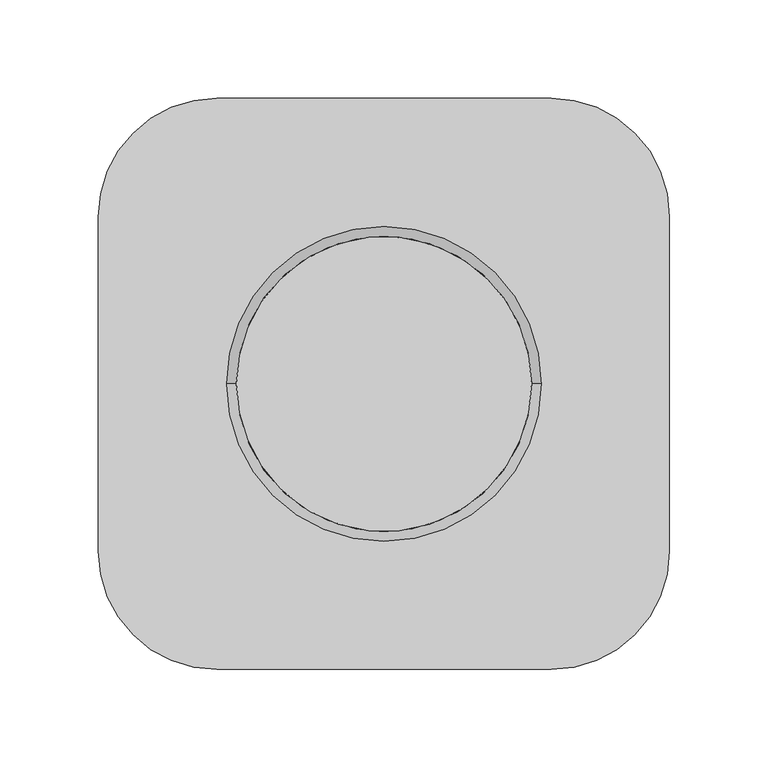
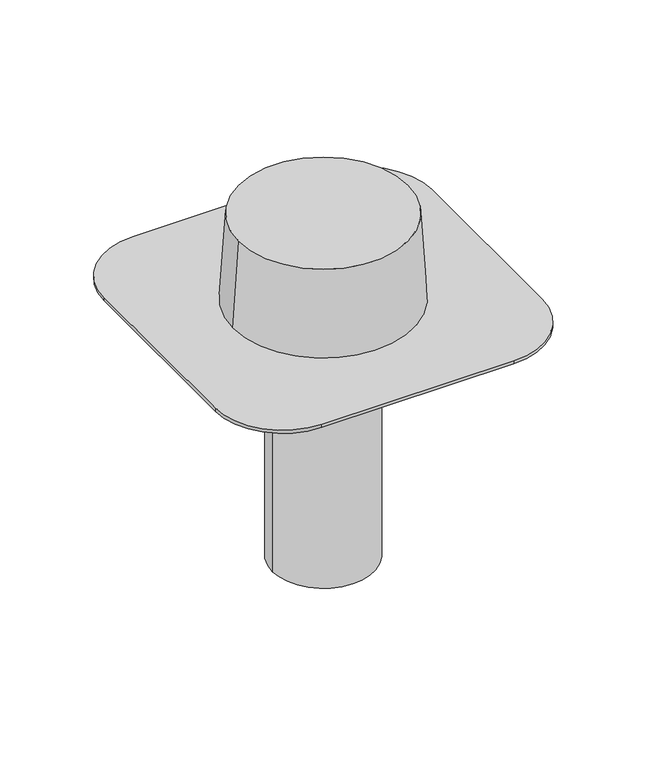
"""IFC4 building model written with IfcOpenShell, lengths in millimetres: proxy geometry, TN_Воронка ТехноНИКОЛЬ ремонтная : Воронка ТехноНИКОЛЬ ремонтная, 90Х240."""

from ifc_helpers import new_model, si_unit, frame, origin, place, context, project, spatial, polyline, circle_curve, source, transform, mapped, element, save
from ifc_brep_helpers import plane_surface, cylinder_surface, revolved_surface, advanced_brep


def specialty_equipment_9be2945b(model_context):
    return source(origin(), model_context, "Body", "AdvancedBrep", [
        advanced_brep(
        [(0.0, 0.0, -240.0), (-45.0, 0.0, -240.0), (45.0, 0.0, -240.0), (-45.0, 0.0, -3.0), (45.0, 0.0, -3.0), (85.0, 145.0, -3.0), (145.0, 85.0, -3.0), (145.0, -85.0, -3.0), (85.0, -145.0, -3.0), (-85.0, -145.0, -3.0), (-145.0, -85.0, -3.0), (-145.0, 85.0, -3.0), (-85.0, 145.0, -3.0), (85.0, 145.0, 0.0), (-85.0, 145.0, 0.0), (-145.0, 85.0, 0.0), (-145.0, -85.0, 0.0), (-85.0, -145.0, 0.0), (85.0, -145.0, 0.0), (145.0, -85.0, 0.0), (145.0, 85.0, 0.0)],
        [
            (0, 1),
            (1, 2, circle_curve(frame((0.0, 0.0, -240.0), z_axis=(0.0, 0.0, -1.0), x_axis=(-1.0, 0.0, 0.0)), 45.0)),
            (2, 0),
            (2, 1, circle_curve(frame((0.0, 0.0, -240.0), z_axis=(0.0, 0.0, -1.0), x_axis=(-1.0, 0.0, 0.0)), 45.0)),
            (1, 3),
            (3, 4, circle_curve(frame((0.0, 0.0, -3.0), z_axis=(0.0, 0.0, -1.0), x_axis=(-1.0, 0.0, 0.0)), 45.0)),
            (4, 2),
            (4, 3, circle_curve(frame((0.0, 0.0, -3.0), z_axis=(0.0, 0.0, -1.0), x_axis=(-1.0, 0.0, 0.0)), 45.0)),
            (5, 6, circle_curve(frame((85.0, 85.0, -3.0), z_axis=(0.0, 0.0, -1.0), x_axis=(1.0, 0.0, 0.0)), 60.0)),
            (6, 7),
            (7, 8, circle_curve(frame((85.0, -85.0, -3.0), z_axis=(0.0, 0.0, -1.0), x_axis=(1.0, 0.0, 0.0)), 60.0)),
            (8, 9),
            (9, 10, circle_curve(frame((-85.0, -85.0, -3.0), z_axis=(0.0, 0.0, -1.0), x_axis=(1.0, 0.0, 0.0)), 60.0)),
            (10, 11),
            (11, 12, circle_curve(frame((-85.0, 85.0, -3.0), z_axis=(0.0, 0.0, -1.0), x_axis=(1.0, 0.0, 0.0)), 60.0)),
            (12, 5),
            (13, 14),
            (14, 15, circle_curve(frame((-85.0, 85.0, 0.0), z_axis=(0.0, 0.0, 1.0), x_axis=(1.0, 0.0, 0.0)), 60.0)),
            (15, 16),
            (16, 17, circle_curve(frame((-85.0, -85.0, 0.0), z_axis=(0.0, 0.0, 1.0), x_axis=(1.0, 0.0, 0.0)), 60.0)),
            (17, 18),
            (18, 19, circle_curve(frame((85.0, -85.0, 0.0), z_axis=(0.0, 0.0, 1.0), x_axis=(1.0, 0.0, 0.0)), 60.0)),
            (19, 20),
            (20, 13, circle_curve(frame((85.0, 85.0, 0.0), z_axis=(0.0, 0.0, 1.0), x_axis=(1.0, 0.0, 0.0)), 60.0)),
            (12, 14),
            (13, 5),
            (10, 16),
            (15, 11),
            (8, 18),
            (17, 9),
            (6, 20),
            (19, 7),
        ],
        [
            plane_surface(frame((0.0, 0.0, -240.0), z_axis=(0.0, 0.0, -1.0), x_axis=(-1.0, 0.0, 0.0))),
            cylinder_surface(frame((0.0, 0.0, 0.0), z_axis=(0.0, 0.0, -1.0), x_axis=(-1.0, 0.0, 0.0)), 45.0),
            plane_surface(frame((-350.0, 145.0, -3.0), z_axis=(0.0, 0.0, -1.0), x_axis=(1.0, 0.0, 0.0))),
            plane_surface(frame((-350.0, 145.0, 0.0), z_axis=(0.0, 0.0, 1.0), x_axis=(-1.0, 0.0, 0.0))),
            plane_surface(frame((85.0, 145.0, 0.0), z_axis=(0.0, 1.0, 0.0), x_axis=(0.0, 0.0, -1.0))),
            plane_surface(frame((-145.0, 85.0, 0.0), z_axis=(-1.0, 0.0, 0.0), x_axis=(0.0, 0.0, -1.0))),
            plane_surface(frame((-85.0, -145.0, 0.0), z_axis=(0.0, -1.0, 0.0), x_axis=(0.0, 0.0, -1.0))),
            plane_surface(frame((145.0, -85.0, 0.0), z_axis=(1.0, 0.0, 0.0), x_axis=(0.0, 0.0, -1.0))),
            cylinder_surface(frame((-85.0, 85.0, -3.0), z_axis=(0.0, 0.0, 1.0), x_axis=(1.0, 0.0, 0.0)), 60.0),
            cylinder_surface(frame((-85.0, -85.0, -3.0), z_axis=(0.0, 0.0, 1.0), x_axis=(1.0, 0.0, 0.0)), 60.0),
            cylinder_surface(frame((85.0, -85.0, -3.0), z_axis=(0.0, 0.0, 1.0), x_axis=(1.0, 0.0, 0.0)), 60.0),
            cylinder_surface(frame((85.0, 85.0, -3.0), z_axis=(0.0, 0.0, 1.0), x_axis=(1.0, 0.0, 0.0)), 60.0),
        ],
        [
            (0, [[1, 2, 3]]),
            (0, [[-1, -3, 4]]),
            (1, [[-2, 5, 6, 7]]),
            (1, [[-4, -7, 8, -5]]),
            (2, [[9, 10, 11, 12, 13, 14, 15, 16], [-6, -8]]),
            (3, [[17, 18, 19, 20, 21, 22, 23, 24]]),
            (4, [[-16, 25, -17, 26]]),
            (5, [[-14, 27, -19, 28]]),
            (6, [[-12, 29, -21, 30]]),
            (7, [[-10, 31, -23, 32]]),
            (8, [[-15, -28, -18, -25]]),
            (9, [[-13, -30, -20, -27]]),
            (10, [[-11, -32, -22, -29]]),
            (11, [[-9, -26, -24, -31]]),
        ],
    ),
        advanced_brep(
        [(-75.0, 0.0, 80.0), (75.0, 0.0, 80.0), (-80.0, 0.0, 0.0), (80.0, 0.0, 0.0)],
        [
            (0, 1, circle_curve(frame((0.0, 0.0, 80.0), z_axis=(0.0, 0.0, 1.0), x_axis=(-1.0, 0.0, 0.0)), 75.0)),
            (1, 0, circle_curve(frame((0.0, 0.0, 80.0), z_axis=(0.0, 0.0, 1.0), x_axis=(1.0, 0.0, 0.0)), 75.0)),
            (2, 3, circle_curve(frame((0.0, 0.0, 0.0), z_axis=(0.0, 0.0, -1.0), x_axis=(1.0, 0.0, 0.0)), 80.0)),
            (3, 2, circle_curve(frame((0.0, 0.0, 0.0), z_axis=(0.0, 0.0, -1.0), x_axis=(-1.0, 0.0, 0.0)), 80.0)),
            (3, 1),
            (0, 2),
        ],
        [
            plane_surface(frame((0.0, 0.0, 80.0), z_axis=(0.0, 0.0, 1.0), x_axis=(0.0, -1.0, 0.0))),
            plane_surface(frame((0.0, 0.0, 0.0), z_axis=(0.0, 0.0, -1.0), x_axis=(0.0, -1.0, 0.0))),
            revolved_surface(polyline([(-75.0, 0.0, 80.0), (-80.0, 0.0, 0.0)]), (0.0, 0.0, 1280.0), (0.0, 0.0, -1.0)),
            revolved_surface(polyline([(75.0, 0.0, 80.0), (80.0, 0.0, 0.0)]), (0.0, 0.0, 1280.0), (0.0, 0.0, -1.0)),
        ],
        [
            (0, [[1, 2]]),
            (1, [[3, 4]]),
            (2, [[-4, 5, -1, 6]]),
            (3, [[-3, -6, -2, -5]]),
        ],
    ),
    ])


if __name__ == "__main__":
    model = new_model("IFC4")
    model_context = context("Model", 3, world=origin())
    ifc_project = project(units=[si_unit("LENGTHUNIT", "METRE", prefix="MILLI")], contexts=[model_context])
    site = spatial("IfcSite", under=ifc_project)
    building = spatial("IfcBuilding", under=site)
    placement = place(None, origin())
    specialty_equipment_shape = specialty_equipment_9be2945b(model_context)
    element("IfcBuildingElementProxy", 1, Name="TN_Воронка ТехноНИКОЛЬ ремонтная : Воронка ТехноНИКОЛЬ ремонтная, 90Х240", ObjectType="TN_Воронка ТехноНИКОЛЬ ремонтная : Воронка ТехноНИКОЛЬ ремонтная, 90Х240", at=placement, inside=building, context=model_context, shape_type="MappedRepresentation", body=[
        mapped(specialty_equipment_shape, transform((0.0, 0.0, 0.0), x_axis=(1.0, 0.0, 0.0), y_axis=(0.0, 1.0, 0.0), z_axis=(0.0, 0.0, 1.0))),
    ])
    save(model, "model.ifc")

# Revit data of these elements
# Type "TN_Воронка ТехноНИКОЛЬ ремонтная : Воронка ТехноНИКОЛЬ ремонтная, 90Х240"
#   ADSK_Группирование = "Комплектующие и воронки"
#   Description = "Ремонтная воронка ТехноНИКОЛЬ применяется для восстановления внутреннего водостока с плоских кровель, имеющих системы водослива со стальными, чугунными Ø100мм или пластмассовыми трубами Ø110мм. Воронки могут устанавливаться в кровлю безогневым способом на мастику герметизирующую № 71. Воронка ТехноНИКОЛЬ ремонтная 90х240 используются при ремонте зданий и сооружений с плоскими кровлями. Применяются в кровлях из битумных и битумно-полимерных рулонных и мастичных материалов с внутренним водостоком. Пропускная способность, 7,6 л/сек."
#   Manufacturer = "ТехноНИКОЛЬ"
#   URL = "https://shop.tn.ru/voronka-tehnonikol-remontnaja-90h240-mm"
#   ADSK_Примечание = ""
#   ADSK_Обозначение = "ТехноНИКОЛЬ"
#   ADSK_Наименование = "Воронка ТехноНИКОЛЬ ремонтная, 90Х240"
#   ADSK_Марка = ""
#   ADSK_Код изделия = "460064"
#   ADSK_Завод-изготовитель = "ТехноНИКОЛЬ"
#   ADSK_Единица измерения = "шт."
#   ADSK_Группирование = "Комплектующие и воронки"
#   ADSK_URL страницы изделия = "https://shop.tn.ru/voronka-tehnonikol-remontnaja-c-uplotnitelem-90h240-mm"
#   ADSK_URL документации изделия = "https://nav.tn.ru/upload/iblock/5b0/Tekhlist-7.22_Voronka_remontnaya_rus.pdf"
#   Пропускная способность = 7.6 L/s
#   Длина расчетная [instance default] = 240 mm
#   Длина отвода [instance default] = 240 mm
#   Диаметр = 90 mm
#   ADSK_Масса = 0.6
#   ADSK_Количество = 1
#   Уплотнитель = no
#   Материал = TN_ПВХ_Черный
#   Default Elevation = 0
# Element 1 (IfcBuildingElementProxy, "TN_Воронка ТехноНИКОЛЬ ремонтная : Воронка ТехноНИКОЛЬ ремонтная, 90Х240")
#   Materials on its faces: "TN_ПВХ_Черный"
# Materials
#   "TN_ПВХ_Черный": class "Типовые", colour RGB 48 48 48, transparency 0, Cost = 0
